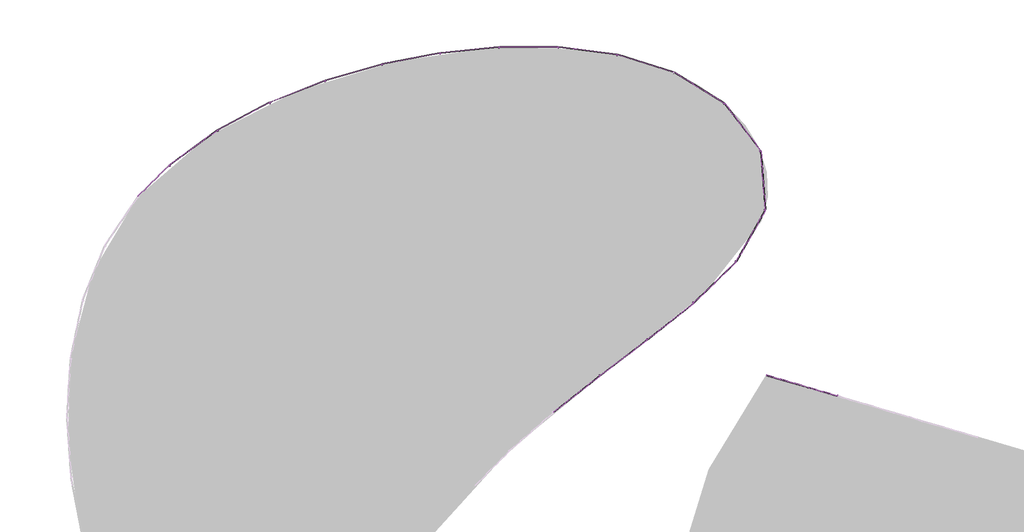
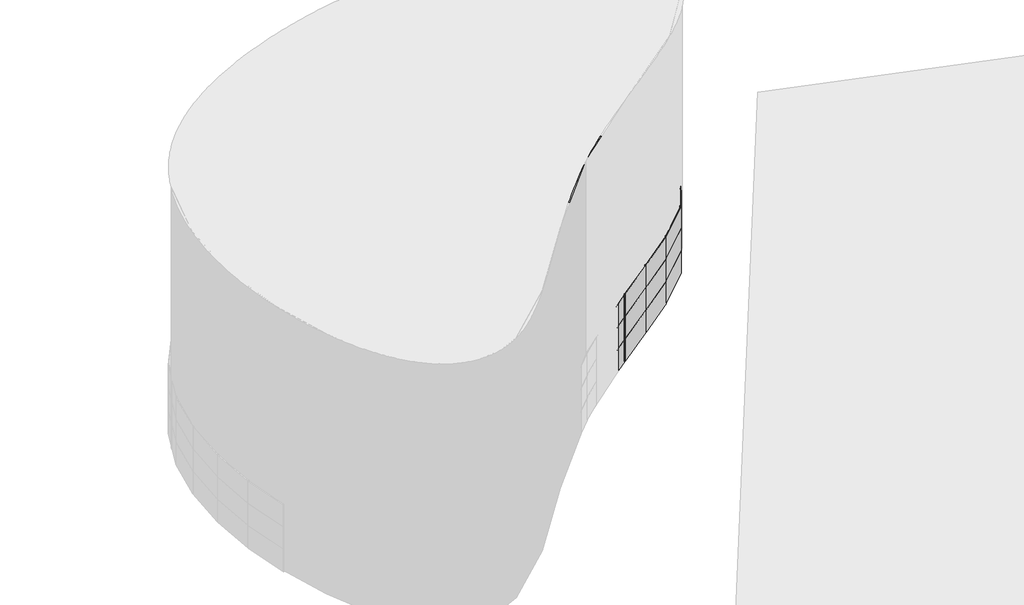
# One storey, part 4 of 5: 59 plates, 53 members.
"""IFC4 building model written with IfcOpenShell, lengths in millimetres."""

import ifcopenshell
import ifcopenshell.guid

model = None  # the IFC model being written
_history = None  # IfcOwnerHistory: only IFC2X3 demands one
_inside = {}  # id of a spatial element -> (the spatial element, [elements in it])
_under = {}  # id of a project, library or spatial element -> (it, [spatial elements below it])
_declared = {}  # id of a project -> (the project, [libraries it declares])
_typed = {}  # id of a type object -> (the type object, [elements of that type])
_made_of = {}  # id of a material, layer set ... -> (it, [elements and type objects made of it])


def new_model(schema):
    """Start an empty IFC model of exactly this schema.

    Asked for "IFC4X3", IfcOpenShell would pick the latest addendum, in which some entities
    have other attributes; the version numbers below select the first issue.
    IFC2X3 requires an IfcOwnerHistory on every rooted entity: one is made here for all.
    """
    global model, _history
    if schema == "IFC4X3":
        model = ifcopenshell.file(schema_version=(4, 3, 0, 0))
    else:
        model = ifcopenshell.file(schema=schema)
    _inside.clear()
    _under.clear()
    _declared.clear()
    _typed.clear()
    _made_of.clear()
    _history = None
    if model.schema == "IFC2X3":
        org = make("IfcOrganization", Name="unknown")
        user = make(
            "IfcPersonAndOrganization",
            ThePerson=make("IfcPerson", FamilyName="unknown"),
            TheOrganization=org,
        )
        app = make(
            "IfcApplication",
            ApplicationDeveloper=org,
            Version="unknown",
            ApplicationFullName="unknown",
            ApplicationIdentifier="unknown",
        )
        _history = make(
            "IfcOwnerHistory",
            OwningUser=user,
            OwningApplication=app,
            ChangeAction="ADDED",
            CreationDate=0,
        )
    return model


def make(cls, **values):
    """One entity of the class cls with the attributes given. An attribute that is None is left unset."""
    return model.create_entity(
        cls, **{name: value for name, value in values.items() if value is not None}
    )


def rooted(cls, **values):
    """An entity with a GlobalId (a new one), such as an element, a storey or a relation."""
    return make(cls, GlobalId=ifcopenshell.guid.new(), OwnerHistory=_history, **values)


def si_unit(unit_type, name, prefix=None):
    """IfcSIUnit, for example si_unit("LENGTHUNIT", "METRE", prefix="MILLI")."""
    return make("IfcSIUnit", UnitType=unit_type, Prefix=prefix, Name=name)


def assignment(units):
    """IfcUnitAssignment: the units of a project."""
    return None if units is None else make("IfcUnitAssignment", Units=units)


def point(xyz):
    """IfcCartesianPoint."""
    return None if xyz is None else make("IfcCartesianPoint", Coordinates=xyz)


def direction(xyz):
    """IfcDirection."""
    return None if xyz is None else make("IfcDirection", DirectionRatios=xyz)


def frame(location, z_axis=None, x_axis=None):
    """IfcAxis2Placement3D, a coordinate frame: its origin and axes. An axis left out is left unset."""
    return make(
        "IfcAxis2Placement3D",
        Location=point(location),
        Axis=direction(z_axis),
        RefDirection=direction(x_axis),
    )


def frame_2d(location, x_axis=None):
    """IfcAxis2Placement2D, a coordinate frame in the plane: its origin and x axis."""
    return make(
        "IfcAxis2Placement2D", Location=point(location), RefDirection=direction(x_axis)
    )


def origin():
    """The frame at (0, 0, 0) with its axes left unset."""
    return frame((0.0, 0.0, 0.0))


def origin_with_axes():
    """The frame at (0, 0, 0) with the z axis (0, 0, 1) and the x axis (1, 0, 0) written out."""
    return frame((0.0, 0.0, 0.0), z_axis=(0.0, 0.0, 1.0), x_axis=(1.0, 0.0, 0.0))


def origin_2d():
    """The frame at (0, 0) in the plane with its x axis left unset."""
    return frame_2d((0.0, 0.0))


def place(relative_to, where):
    """IfcLocalPlacement: puts the frame where relative to a parent placement (None: the world)."""
    return make(
        "IfcLocalPlacement", PlacementRelTo=relative_to, RelativePlacement=where
    )


def context(
    kind, dimensions, precision=None, world=None, true_north=None, identifier=None
):
    """IfcGeometricRepresentationContext, for example the 3D "Model" context."""
    return make(
        "IfcGeometricRepresentationContext",
        ContextIdentifier=identifier,
        ContextType=kind,
        CoordinateSpaceDimension=dimensions,
        Precision=precision,
        WorldCoordinateSystem=world,
        TrueNorth=true_north,
    )


def project(units=None, contexts=None):
    """IfcProject with its units and contexts."""
    return rooted(
        "IfcProject",
        Name="project",
        RepresentationContexts=contexts,
        UnitsInContext=assignment(units),
    )


def spatial(cls, under=None, at=None, **own):
    """A site, building, storey or space (cls), placed at a placement, below another one or the project."""
    s = rooted(cls, ObjectPlacement=at, **own)
    if under is not None:
        _under.setdefault(under.id(), (under, []))[1].append(s)
    return s


def polyline(points):
    """IfcPolyline through the points."""
    return make("IfcPolyline", Points=[point(p) for p in points])


def circle_curve(where, radius):
    """IfcCircle in the frame where."""
    return make("IfcCircle", Position=where, Radius=radius)


def trimmed(basis, trim1, trim2, sense, master):
    """IfcTrimmedCurve: the piece of a basis curve between two trims."""
    return make(
        "IfcTrimmedCurve",
        BasisCurve=basis,
        Trim1=trim1,
        Trim2=trim2,
        SenseAgreement=sense,
        MasterRepresentation=master,
    )


def segment(curve, same_sense, transition):
    """IfcCompositeCurveSegment."""
    return make(
        "IfcCompositeCurveSegment",
        Transition=transition,
        SameSense=same_sense,
        ParentCurve=curve,
    )


def composite_curve(segments, self_intersect=None):
    """IfcCompositeCurve: segments joined end to end."""
    return make("IfcCompositeCurve", Segments=segments, SelfIntersect=self_intersect)


def outline(outer, holes=None, kind="AREA"):
    """IfcArbitraryClosedProfileDef: a profile drawn as a closed curve; with holes, ...WithVoids."""
    if holes is None:
        return make("IfcArbitraryClosedProfileDef", ProfileType=kind, OuterCurve=outer)
    return make(
        "IfcArbitraryProfileDefWithVoids",
        ProfileType=kind,
        OuterCurve=outer,
        InnerCurves=holes,
    )


def extrude(swept, where, along, depth):
    """IfcExtrudedAreaSolid: the profile swept, set in the frame where, extruded along a direction by depth."""
    return make(
        "IfcExtrudedAreaSolid",
        SweptArea=swept,
        Position=where,
        ExtrudedDirection=direction(along),
        Depth=depth,
    )


def shape(context_of_items, identifier, shape_type, items):
    """IfcShapeRepresentation: the items that make up one representation, for example the "Body"."""
    return make(
        "IfcShapeRepresentation",
        ContextOfItems=context_of_items,
        RepresentationIdentifier=identifier,
        RepresentationType=shape_type,
        Items=items,
    )


def source(mapping_origin, context_of_items, identifier, shape_type, items):
    """IfcRepresentationMap: a shape defined once, which mapped items show again and again."""
    return make(
        "IfcRepresentationMap",
        MappingOrigin=mapping_origin,
        MappedRepresentation=shape(context_of_items, identifier, shape_type, items),
    )


def transform(
    local_origin,
    x_axis=None,
    y_axis=None,
    z_axis=None,
    scale=None,
    scale2=None,
    scale3=None,
    uniform=True,
):
    """IfcCartesianTransformationOperator3D, or its non-uniform kind. x_axis, y_axis, z_axis: its Axis1, 2, 3."""
    if uniform:
        return make(
            "IfcCartesianTransformationOperator3D",
            Axis1=direction(x_axis),
            Axis2=direction(y_axis),
            LocalOrigin=point(local_origin),
            Scale=scale,
            Axis3=direction(z_axis),
        )
    return make(
        "IfcCartesianTransformationOperator3DnonUniform",
        Axis1=direction(x_axis),
        Axis2=direction(y_axis),
        LocalOrigin=point(local_origin),
        Scale=scale,
        Axis3=direction(z_axis),
        Scale2=scale2,
        Scale3=scale3,
    )


def mapped(mapping_source, mapping_target):
    """IfcMappedItem: shows the shape of a source again, moved by a transform."""
    return make(
        "IfcMappedItem", MappingSource=mapping_source, MappingTarget=mapping_target
    )


def made_of(thing, what):
    """Note that an element or type object is made of a material, layer set ...; save() writes the relation."""
    if what is not None:
        _made_of.setdefault(what.id(), (what, []))[1].append(thing)
    return thing


def element(
    cls,
    number,
    at=None,
    inside=None,
    cuts=None,
    type_object=None,
    material=None,
    context=None,
    identifier="Body",
    shape_type=None,
    held_by="IfcProductDefinitionShape",
    body=None,
    shapes=None,
    **own,
):
    """One element of the class cls, such as IfcWall. Its Tag is "e" and its number.

    at: its placement. inside: the storey or other place that contains it. cuts: it is an
    opening in that element (IfcRelVoidsElement). A single representation is given by context,
    identifier, shape_type and body (its items); several are given by shapes. held_by: the class
    of the entity that holds the representations. save() writes the other relations.
    """
    e = rooted(cls, Tag="e%d" % number, ObjectPlacement=at, **own)
    if body is not None:
        shapes = [shape(context, identifier, shape_type, body)]
    if shapes is not None:
        e.Representation = make(held_by, Representations=shapes)
    if inside is not None:
        _inside.setdefault(inside.id(), (inside, []))[1].append(e)
    if cuts is not None:
        rooted(
            "IfcRelVoidsElement", RelatingBuildingElement=cuts, RelatedOpeningElement=e
        )
    if type_object is not None:
        _typed.setdefault(type_object.id(), (type_object, []))[1].append(e)
    return made_of(e, material)


def aggregate(whole, parts):
    """IfcRelAggregates: a whole, such as a stair, and the parts it consists of."""
    return rooted("IfcRelAggregates", RelatingObject=whole, RelatedObjects=parts)


def save(model, path):
    """Write the relations noted so far, then the file.

    IfcRelAggregates (storeys below a building ...), IfcRelContainedInSpatialStructure (elements
    in a storey), IfcRelDefinesByType, IfcRelAssociatesMaterial and IfcRelDeclares: one each for
    every whole, place, type object, material and project.
    """
    for whole, parts in _under.values():
        aggregate(whole, parts)
    for where, things in _inside.values():
        rooted(
            "IfcRelContainedInSpatialStructure",
            RelatedElements=things,
            RelatingStructure=where,
        )
    for kind, things in _typed.values():
        rooted("IfcRelDefinesByType", RelatedObjects=things, RelatingType=kind)
    for what, things in _made_of.values():
        rooted("IfcRelAssociatesMaterial", RelatedObjects=things, RelatingMaterial=what)
    for by, libraries in _declared.values():
        rooted("IfcRelDeclares", RelatingContext=by, RelatedDefinitions=libraries)
    model.write(path)


def montante_circular_25_mm_raio_36e581cf(model_context):
    return source(origin(), model_context, "Body", "SweptSolid", [
        extrude(outline(composite_curve([segment(trimmed(circle_curve(origin_2d(), 25.0), [point((25.0, 0.0))], [point((-25.0, 0.0))], False, "CARTESIAN"), True, "CONTINUOUS"), segment(trimmed(circle_curve(origin_2d(), 25.0), [point((-25.0, 0.0))], [point((25.0, 0.0))], False, "CARTESIAN"), True, "CONTINUOUS")], self_intersect=False)), frame((0.0, 0.0, -1500.0), z_axis=(0.0, 0.0, 1.0), x_axis=(1.0, 0.0, 0.0)), (0.0, 0.0, 1.0), 1500.0),
    ])


def montante_circular_25_mm_raio_a1f35a82(model_context):
    return source(origin(), model_context, "Body", "SweptSolid", [
        extrude(outline(composite_curve([segment(trimmed(circle_curve(origin_2d(), 25.0), [point((25.0, 0.0))], [point((-25.0, 0.0))], False, "CARTESIAN"), True, "CONTINUOUS"), segment(trimmed(circle_curve(origin_2d(), 25.0), [point((-25.0, 0.0))], [point((25.0, 0.0))], False, "CARTESIAN"), True, "CONTINUOUS")], self_intersect=False)), frame((0.0, 0.0, -727.4383788), z_axis=(0.0, 0.0, 1.0), x_axis=(1.0, 0.0, 0.0)), (0.0, 0.0, 1.0), 727.4383788),
    ])


def painel_do_sistema_ee4f1c4d(model_context):
    return source(origin(), model_context, "Body", "SweptSolid", [
        extrude(outline(polyline([(1487.5000075, 24.5), (-1487.5000075, 24.5), (-1487.5000075, 49.5), (1487.5000075, 49.5), (1487.5000075, 24.5)])), origin_with_axes(), (0.0, 0.0, 1.0), 1500.0),
    ])


def painel_do_sistema_5ef9eced(model_context):
    return source(origin(), model_context, "Body", "SweptSolid", [
        extrude(outline(polyline([(1475.0, 24.5), (-1475.0, 24.5), (-1475.0, 49.5), (1475.0, 49.5), (1475.0, 24.5)])), origin_with_axes(), (0.0, 0.0, 1.0), 1500.0),
    ])


def painel_do_sistema_cd1f443e(model_context):
    return source(origin(), model_context, "Body", "SweptSolid", [
        extrude(outline(polyline([(1487.5000075, 24.5), (-1487.5000075, 24.5), (-1487.5000075, 49.5), (1487.5000075, 49.5), (1487.5000075, 24.5)])), origin_with_axes(), (0.0, 0.0, 1.0), 727.4383788),
    ])


def painel_do_sistema_bf426e09(model_context):
    return source(origin(), model_context, "Body", "SweptSolid", [
        extrude(outline(polyline([(1475.0, 24.5), (-1475.0, 24.5), (-1475.0, 49.5), (1475.0, 49.5), (1475.0, 24.5)])), origin_with_axes(), (0.0, 0.0, 1.0), 727.4383788),
    ])


def painel_do_sistema_85ccde5d(model_context):
    return source(origin(), model_context, "Body", "SweptSolid", [
        extrude(outline(polyline([(1475.0, -49.5), (-1475.0, -49.5), (-1475.0, -24.5), (1475.0, -24.5), (1475.0, -49.5)])), origin_with_axes(), (0.0, 0.0, 1.0), 1500.0),
    ])


def painel_do_sistema_91df381f(model_context):
    return source(origin(), model_context, "Body", "SweptSolid", [
        extrude(outline(polyline([(1110.3819696, -49.5), (-1110.3819696, -49.5), (-1110.3819696, -24.5), (1110.3819696, -24.5), (1110.3819696, -49.5)])), origin_with_axes(), (0.0, 0.0, 1.0), 1500.0),
    ])


model = new_model("IFC4")

# Units and contexts
model_context = context("Model", 3, world=origin())
ifc_project = project(units=[si_unit("LENGTHUNIT", "METRE", prefix="MILLI")], contexts=[model_context])

# Site, building, storey
site = spatial("IfcSite", under=ifc_project)
building = spatial("IfcBuilding", under=site)
storey = spatial("IfcBuildingStorey", under=building, Name="Nível 1", Elevation=0.0)

# Members
placement = place(None, origin())
montante_circular_25_mm_raio_shape = montante_circular_25_mm_raio_36e581cf(model_context)
element("IfcMember", 1, ObjectType="Montante circular : 25 mm Raio", at=placement, inside=storey, context=model_context, shape_type="MappedRepresentation", body=[
    mapped(montante_circular_25_mm_raio_shape, transform((-4389.7681283, 32366.1480949, 3000.000015), x_axis=(0.0, 0.0, 1.0), y_axis=(0.28318378939534594, 0.95906566064253, 0.0), z_axis=(-0.95906566064253, 0.28318378939534594, 0.0))),
])
element("IfcMember", 2, ObjectType="Montante circular : 25 mm Raio", at=placement, inside=storey, context=model_context, shape_type="MappedRepresentation", body=[
    mapped(montante_circular_25_mm_raio_shape, transform((-5828.3666192, 32790.923779, 3000.000015), x_axis=(0.0, 0.0, 1.0), y_axis=(0.283183789395347, 0.9590656606425296, 0.0), z_axis=(-0.9590656606425296, 0.283183789395347, 0.0))),
])
element("IfcMember", 3, ObjectType="Montante circular : 25 mm Raio", at=placement, inside=storey, context=model_context, shape_type="MappedRepresentation", body=[
    mapped(montante_circular_25_mm_raio_shape, transform((-14996.1891623, 32974.6356945, 1500.0), x_axis=(0.7952150611070873, 0.6063274747102028, 0.0), y_axis=(0.6063274747102028, -0.7952150611070873, 0.0), z_axis=(0.0, 0.0, -1.0))),
])
element("IfcMember", 4, ObjectType="Montante circular : 25 mm Raio", at=placement, inside=storey, context=model_context, shape_type="MappedRepresentation", body=[
    mapped(montante_circular_25_mm_raio_shape, transform((-12604.1298635, 34785.1749266, 1500.0), x_axis=(0.7953870623365296, 0.6061018240095187, 0.0), y_axis=(0.6061018240095187, -0.7953870623365296, 0.0), z_axis=(0.0, 0.0, -1.0))),
])
element("IfcMember", 5, ObjectType="Montante circular : 25 mm Raio", at=placement, inside=storey, context=model_context, shape_type="MappedRepresentation", body=[
    mapped(montante_circular_25_mm_raio_shape, transform((-10255.474771, 36651.6741247, 1500.0), x_axis=(0.7627263023971693, 0.6467214142361005, 0.0), y_axis=(0.6467214142361005, -0.7627263023971693, 0.0), z_axis=(0.0, 0.0, -1.0))),
])
element("IfcMember", 6, ObjectType="Montante circular : 25 mm Raio", at=placement, inside=storey, context=model_context, shape_type="MappedRepresentation", body=[
    mapped(montante_circular_25_mm_raio_shape, transform((-8101.871437, 38740.2125323, 1500.0), x_axis=(0.6490334571140041, 0.7607598645739958, 0.0), y_axis=(0.7607598645739958, -0.6490334571140041, 0.0), z_axis=(0.0, 0.0, -1.0))),
])
element("IfcMember", 7, ObjectType="Montante circular : 25 mm Raio", at=placement, inside=storey, context=model_context, shape_type="MappedRepresentation", body=[
    mapped(montante_circular_25_mm_raio_shape, transform((-6627.5874319, 41352.9671461, 1500.0), x_axis=(0.24827563424230142, 0.9686894287859155, 0.0), y_axis=(0.9686894287859155, -0.24827563424230142, 0.0), z_axis=(0.0, 0.0, -1.0))),
])
element("IfcMember", 8, ObjectType="Montante circular : 25 mm Raio", at=placement, inside=storey, context=model_context, shape_type="MappedRepresentation", body=[
    mapped(montante_circular_25_mm_raio_shape, transform((-6868.5829053, 44343.271676, 1500.0), x_axis=(-0.3894872634933398, 0.9210318515537178, 0.0), y_axis=(0.9210318515537178, 0.3894872634933398, 0.0), z_axis=(0.0, 0.0, -1.0))),
])
element("IfcMember", 9, ObjectType="Montante circular : 25 mm Raio", at=placement, inside=storey, context=model_context, shape_type="MappedRepresentation", body=[
    mapped(montante_circular_25_mm_raio_shape, transform((-8685.5307871, 46730.4667655, 1500.0), x_axis=(-0.7608105002607383, 0.6489741001711895, 0.0), y_axis=(0.6489741001711895, 0.7608105002607383, 0.0), z_axis=(0.0, 0.0, -1.0))),
])
element("IfcMember", 10, ObjectType="Montante circular : 25 mm Raio", at=placement, inside=storey, context=model_context, shape_type="MappedRepresentation", body=[
    mapped(montante_circular_25_mm_raio_shape, transform((-11244.034472, 48297.0103794, 1500.0), x_axis=(-0.9160451113541028, 0.40107524725947563, 0.0), y_axis=(0.40107524725947563, 0.9160451113541028, 0.0), z_axis=(0.0, 0.0, -1.0))),
])
element("IfcMember", 11, ObjectType="Montante circular : 25 mm Raio", at=placement, inside=storey, context=model_context, shape_type="MappedRepresentation", body=[
    mapped(montante_circular_25_mm_raio_shape, transform((-14105.1754803, 49199.1589981, 1500.0), x_axis=(-0.9782677823869713, 0.20734547485700602, 0.0), y_axis=(0.20734547485700602, 0.9782677823869713, 0.0), z_axis=(0.0, 0.0, -1.0))),
])
element("IfcMember", 12, ObjectType="Montante circular : 25 mm Raio", at=placement, inside=storey, context=model_context, shape_type="MappedRepresentation", body=[
    mapped(montante_circular_25_mm_raio_shape, transform((-17080.2416106, 49585.140242, 1500.0), x_axis=(-0.998380379517221, 0.05689128048347721, 0.0), y_axis=(0.05689128048347721, 0.998380379517221, 0.0), z_axis=(0.0, 0.0, -1.0))),
])
element("IfcMember", 13, ObjectType="Montante circular : 25 mm Raio", at=placement, inside=storey, context=model_context, shape_type="MappedRepresentation", body=[
    mapped(montante_circular_25_mm_raio_shape, transform((-20080.239517, 49581.5960042, 1500.0), x_axis=(-0.9985092878419478, -0.054582067507252724, 0.0), y_axis=(-0.054582067507252724, 0.9985092878419478, 0.0), z_axis=(0.0, 0.0, -1.0))),
])
element("IfcMember", 14, ObjectType="Montante circular : 25 mm Raio", at=placement, inside=storey, context=model_context, shape_type="MappedRepresentation", body=[
    mapped(montante_circular_25_mm_raio_shape, transform((-23064.637889, 49276.0369149, 1500.0), x_axis=(-0.989112077587023, -0.14716418712269305, 0.0), y_axis=(-0.14716418712269305, 0.989112077587023, 0.0), z_axis=(0.0, 0.0, -1.0))),
])
element("IfcMember", 15, ObjectType="Montante circular : 25 mm Raio", at=placement, inside=storey, context=model_context, shape_type="MappedRepresentation", body=[
    mapped(montante_circular_25_mm_raio_shape, transform((-26009.7169515, 48704.6269783, 1500.0), x_axis=(-0.9724041864044524, -0.23330258949076227, 0.0), y_axis=(-0.23330258949076227, 0.9724041864044524, 0.0), z_axis=(0.0, 0.0, -1.0))),
])
element("IfcMember", 16, ObjectType="Montante circular : 25 mm Raio", at=placement, inside=storey, context=model_context, shape_type="MappedRepresentation", body=[
    mapped(montante_circular_25_mm_raio_shape, transform((-28892.5410808, 47874.3709699, 1500.0), x_axis=(-0.947152921337535, -0.3207823929111028, 0.0), y_axis=(-0.3207823929111028, 0.947152921337535, 0.0), z_axis=(0.0, 0.0, -1.0))),
])
element("IfcMember", 17, ObjectType="Montante circular : 25 mm Raio", at=placement, inside=storey, context=model_context, shape_type="MappedRepresentation", body=[
    mapped(montante_circular_25_mm_raio_shape, transform((-31682.4252949, 46771.3994961, 1500.0), x_axis=(-0.9093535544571357, -0.4160241735718888, 0.0), y_axis=(-0.4160241735718888, 0.9093535544571357, 0.0), z_axis=(0.0, 0.0, -1.0))),
])
element("IfcMember", 18, ObjectType="Montante circular : 25 mm Raio", at=placement, inside=storey, context=model_context, shape_type="MappedRepresentation", body=[
    mapped(montante_circular_25_mm_raio_shape, transform((-34331.1697585, 45362.7999198, 1500.0), x_axis=(-0.8509275894835548, -0.5252830070121313, 0.0), y_axis=(-0.5252830070121313, 0.8509275894835548, 0.0), z_axis=(0.0, 0.0, -1.0))),
])
element("IfcMember", 19, ObjectType="Montante circular : 25 mm Raio", at=placement, inside=storey, context=model_context, shape_type="MappedRepresentation", body=[
    mapped(montante_circular_25_mm_raio_shape, transform((-36756.8303499, 43597.5320378, 1500.0), x_axis=(-0.7567414762597636, -0.6537142633507346, 0.0), y_axis=(-0.6537142633507346, 0.7567414762597636, 0.0), z_axis=(0.0, 0.0, -1.0))),
])
element("IfcMember", 20, ObjectType="Montante circular : 25 mm Raio", at=placement, inside=storey, context=model_context, shape_type="MappedRepresentation", body=[
    mapped(montante_circular_25_mm_raio_shape, transform((-14996.1891623, 32974.6356945, 3000.0), x_axis=(0.7952150611070874, 0.6063274747102025, 0.0), y_axis=(0.6063274747102025, -0.7952150611070874, 0.0), z_axis=(0.0, 0.0, -1.0))),
])
element("IfcMember", 21, ObjectType="Montante circular : 25 mm Raio", at=placement, inside=storey, context=model_context, shape_type="MappedRepresentation", body=[
    mapped(montante_circular_25_mm_raio_shape, transform((-12604.1298635, 34785.1749266, 3000.0), x_axis=(0.7953870623365296, 0.6061018240095187, 0.0), y_axis=(0.6061018240095187, -0.7953870623365296, 0.0), z_axis=(0.0, 0.0, -1.0))),
])
element("IfcMember", 22, ObjectType="Montante circular : 25 mm Raio", at=placement, inside=storey, context=model_context, shape_type="MappedRepresentation", body=[
    mapped(montante_circular_25_mm_raio_shape, transform((-10255.474771, 36651.6741247, 3000.0), x_axis=(0.7627263023971692, 0.6467214142361006, 0.0), y_axis=(0.6467214142361006, -0.7627263023971692, 0.0), z_axis=(0.0, 0.0, -1.0))),
])
element("IfcMember", 23, ObjectType="Montante circular : 25 mm Raio", at=placement, inside=storey, context=model_context, shape_type="MappedRepresentation", body=[
    mapped(montante_circular_25_mm_raio_shape, transform((-8101.871437, 38740.2125323, 3000.0), x_axis=(0.6490334571140043, 0.7607598645739955, 0.0), y_axis=(0.7607598645739955, -0.6490334571140043, 0.0), z_axis=(0.0, 0.0, -1.0))),
])
element("IfcMember", 24, ObjectType="Montante circular : 25 mm Raio", at=placement, inside=storey, context=model_context, shape_type="MappedRepresentation", body=[
    mapped(montante_circular_25_mm_raio_shape, transform((-6627.5874319, 41352.9671461, 3000.0), x_axis=(0.24827563424230142, 0.9686894287859154, 0.0), y_axis=(0.9686894287859154, -0.24827563424230142, 0.0), z_axis=(0.0, 0.0, -1.0))),
])
element("IfcMember", 25, ObjectType="Montante circular : 25 mm Raio", at=placement, inside=storey, context=model_context, shape_type="MappedRepresentation", body=[
    mapped(montante_circular_25_mm_raio_shape, transform((-6868.5829053, 44343.271676, 3000.0), x_axis=(-0.3894872634933398, 0.9210318515537178, 0.0), y_axis=(0.9210318515537178, 0.3894872634933398, 0.0), z_axis=(0.0, 0.0, -1.0))),
])
element("IfcMember", 26, ObjectType="Montante circular : 25 mm Raio", at=placement, inside=storey, context=model_context, shape_type="MappedRepresentation", body=[
    mapped(montante_circular_25_mm_raio_shape, transform((-8685.5307871, 46730.4667655, 3000.0), x_axis=(-0.7608105002607387, 0.6489741001711892, 0.0), y_axis=(0.6489741001711892, 0.7608105002607387, 0.0), z_axis=(0.0, 0.0, -1.0))),
])
element("IfcMember", 27, ObjectType="Montante circular : 25 mm Raio", at=placement, inside=storey, context=model_context, shape_type="MappedRepresentation", body=[
    mapped(montante_circular_25_mm_raio_shape, transform((-14105.1754803, 49199.1589981, 3000.0), x_axis=(-0.9782677823869713, 0.20734547485700608, 0.0), y_axis=(0.20734547485700608, 0.9782677823869713, 0.0), z_axis=(0.0, 0.0, -1.0))),
])
element("IfcMember", 28, ObjectType="Montante circular : 25 mm Raio", at=placement, inside=storey, context=model_context, shape_type="MappedRepresentation", body=[
    mapped(montante_circular_25_mm_raio_shape, transform((-17080.2416106, 49585.140242, 3000.0), x_axis=(-0.998380379517221, 0.0568912804834772, 0.0), y_axis=(0.0568912804834772, 0.998380379517221, 0.0), z_axis=(0.0, 0.0, -1.0))),
])
element("IfcMember", 29, ObjectType="Montante circular : 25 mm Raio", at=placement, inside=storey, context=model_context, shape_type="MappedRepresentation", body=[
    mapped(montante_circular_25_mm_raio_shape, transform((-20080.239517, 49581.5960042, 3000.0), x_axis=(-0.9985092878419478, -0.05458206750725284, 0.0), y_axis=(-0.05458206750725284, 0.9985092878419478, 0.0), z_axis=(0.0, 0.0, -1.0))),
])
element("IfcMember", 30, ObjectType="Montante circular : 25 mm Raio", at=placement, inside=storey, context=model_context, shape_type="MappedRepresentation", body=[
    mapped(montante_circular_25_mm_raio_shape, transform((-23064.637889, 49276.0369149, 3000.0), x_axis=(-0.9891120775870231, -0.1471641871226927, 0.0), y_axis=(-0.1471641871226927, 0.9891120775870231, 0.0), z_axis=(0.0, 0.0, -1.0))),
])
element("IfcMember", 31, ObjectType="Montante circular : 25 mm Raio", at=placement, inside=storey, context=model_context, shape_type="MappedRepresentation", body=[
    mapped(montante_circular_25_mm_raio_shape, transform((-26009.7169515, 48704.6269783, 3000.0), x_axis=(-0.9724041864044525, -0.23330258949076174, 0.0), y_axis=(-0.23330258949076174, 0.9724041864044525, 0.0), z_axis=(0.0, 0.0, -1.0))),
])
element("IfcMember", 32, ObjectType="Montante circular : 25 mm Raio", at=placement, inside=storey, context=model_context, shape_type="MappedRepresentation", body=[
    mapped(montante_circular_25_mm_raio_shape, transform((-28892.5410808, 47874.3709699, 3000.0), x_axis=(-0.9471529213375351, -0.3207823929111028, 0.0), y_axis=(-0.3207823929111028, 0.9471529213375351, 0.0), z_axis=(0.0, 0.0, -1.0))),
])
element("IfcMember", 33, ObjectType="Montante circular : 25 mm Raio", at=placement, inside=storey, context=model_context, shape_type="MappedRepresentation", body=[
    mapped(montante_circular_25_mm_raio_shape, transform((-31682.4252949, 46771.3994961, 3000.0), x_axis=(-0.9093535544571357, -0.41602417357188887, 0.0), y_axis=(-0.41602417357188887, 0.9093535544571357, 0.0), z_axis=(0.0, 0.0, -1.0))),
])
element("IfcMember", 34, ObjectType="Montante circular : 25 mm Raio", at=placement, inside=storey, context=model_context, shape_type="MappedRepresentation", body=[
    mapped(montante_circular_25_mm_raio_shape, transform((-34331.1697585, 45362.7999198, 3000.0), x_axis=(-0.850927589483555, -0.5252830070121313, 0.0), y_axis=(-0.5252830070121313, 0.850927589483555, 0.0), z_axis=(0.0, 0.0, -1.0))),
])
element("IfcMember", 35, ObjectType="Montante circular : 25 mm Raio", at=placement, inside=storey, context=model_context, shape_type="MappedRepresentation", body=[
    mapped(montante_circular_25_mm_raio_shape, transform((-36756.8303499, 43597.5320378, 3000.0), x_axis=(-0.7567414762597636, -0.6537142633507346, 0.0), y_axis=(-0.6537142633507346, 0.7567414762597636, 0.0), z_axis=(0.0, 0.0, -1.0))),
])
montante_circular_25_mm_raio_2_shape = montante_circular_25_mm_raio_a1f35a82(model_context)
element("IfcMember", 36, ObjectType="Montante circular : 25 mm Raio", at=placement, inside=storey, context=model_context, shape_type="MappedRepresentation", body=[
    mapped(montante_circular_25_mm_raio_2_shape, transform((-6526.0277886, 32996.9225357, 3000.000015), x_axis=(0.0, 0.0, 1.0), y_axis=(0.28318378939534294, 0.9590656606425308, 0.0), z_axis=(-0.9590656606425308, 0.28318378939534294, 0.0))),
])
element("IfcMember", 37, ObjectType="Montante circular : 25 mm Raio", at=placement, inside=storey, context=model_context, shape_type="MappedRepresentation", body=[
    mapped(montante_circular_25_mm_raio_shape, transform((-14996.1891623, 32974.6356945, 0.0), x_axis=(0.7952150611070873, 0.6063274747102028, 0.0), y_axis=(0.6063274747102028, -0.7952150611070873, 0.0), z_axis=(0.0, 0.0, -1.0))),
])
element("IfcMember", 38, ObjectType="Montante circular : 25 mm Raio", at=placement, inside=storey, context=model_context, shape_type="MappedRepresentation", body=[
    mapped(montante_circular_25_mm_raio_shape, transform((-12604.1298635, 34785.1749266, 0.0), x_axis=(0.7953870623365296, 0.6061018240095187, 0.0), y_axis=(0.6061018240095187, -0.7953870623365296, 0.0), z_axis=(0.0, 0.0, -1.0))),
])
element("IfcMember", 39, ObjectType="Montante circular : 25 mm Raio", at=placement, inside=storey, context=model_context, shape_type="MappedRepresentation", body=[
    mapped(montante_circular_25_mm_raio_shape, transform((-10255.474771, 36651.6741247, 0.0), x_axis=(0.7627263023971693, 0.6467214142361005, 0.0), y_axis=(0.6467214142361005, -0.7627263023971693, 0.0), z_axis=(0.0, 0.0, -1.0))),
])
element("IfcMember", 40, ObjectType="Montante circular : 25 mm Raio", at=placement, inside=storey, context=model_context, shape_type="MappedRepresentation", body=[
    mapped(montante_circular_25_mm_raio_shape, transform((-8101.871437, 38740.2125323, 0.0), x_axis=(0.6490334571140042, 0.7607598645739956, 0.0), y_axis=(0.7607598645739956, -0.6490334571140042, 0.0), z_axis=(0.0, 0.0, -1.0))),
])
element("IfcMember", 41, ObjectType="Montante circular : 25 mm Raio", at=placement, inside=storey, context=model_context, shape_type="MappedRepresentation", body=[
    mapped(montante_circular_25_mm_raio_shape, transform((-6627.5874319, 41352.9671461, 0.0), x_axis=(0.24827563424230142, 0.9686894287859154, 0.0), y_axis=(0.9686894287859154, -0.24827563424230142, 0.0), z_axis=(0.0, 0.0, -1.0))),
])
element("IfcMember", 42, ObjectType="Montante circular : 25 mm Raio", at=placement, inside=storey, context=model_context, shape_type="MappedRepresentation", body=[
    mapped(montante_circular_25_mm_raio_shape, transform((-6868.5829053, 44343.271676, 0.0), x_axis=(-0.3894872634933398, 0.9210318515537178, 0.0), y_axis=(0.9210318515537178, 0.3894872634933398, 0.0), z_axis=(0.0, 0.0, -1.0))),
])
element("IfcMember", 43, ObjectType="Montante circular : 25 mm Raio", at=placement, inside=storey, context=model_context, shape_type="MappedRepresentation", body=[
    mapped(montante_circular_25_mm_raio_shape, transform((-8685.5307871, 46730.4667655, 0.0), x_axis=(-0.7608105002607386, 0.6489741001711892, 0.0), y_axis=(0.6489741001711892, 0.7608105002607386, 0.0), z_axis=(0.0, 0.0, -1.0))),
])
element("IfcMember", 44, ObjectType="Montante circular : 25 mm Raio", at=placement, inside=storey, context=model_context, shape_type="MappedRepresentation", body=[
    mapped(montante_circular_25_mm_raio_shape, transform((-11244.034472, 48297.0103794, 0.0), x_axis=(-0.9160451113541028, 0.40107524725947563, 0.0), y_axis=(0.40107524725947563, 0.9160451113541028, 0.0), z_axis=(0.0, 0.0, -1.0))),
])
element("IfcMember", 45, ObjectType="Montante circular : 25 mm Raio", at=placement, inside=storey, context=model_context, shape_type="MappedRepresentation", body=[
    mapped(montante_circular_25_mm_raio_shape, transform((-14105.1754803, 49199.1589981, 0.0), x_axis=(-0.9782677823869713, 0.20734547485700608, 0.0), y_axis=(0.20734547485700608, 0.9782677823869713, 0.0), z_axis=(0.0, 0.0, -1.0))),
])
element("IfcMember", 46, ObjectType="Montante circular : 25 mm Raio", at=placement, inside=storey, context=model_context, shape_type="MappedRepresentation", body=[
    mapped(montante_circular_25_mm_raio_shape, transform((-17080.2416106, 49585.140242, 0.0), x_axis=(-0.998380379517221, 0.0568912804834772, 0.0), y_axis=(0.0568912804834772, 0.998380379517221, 0.0), z_axis=(0.0, 0.0, -1.0))),
])
element("IfcMember", 47, ObjectType="Montante circular : 25 mm Raio", at=placement, inside=storey, context=model_context, shape_type="MappedRepresentation", body=[
    mapped(montante_circular_25_mm_raio_shape, transform((-20080.239517, 49581.5960042, 0.0), x_axis=(-0.9985092878419478, -0.05458206750725284, 0.0), y_axis=(-0.05458206750725284, 0.9985092878419478, 0.0), z_axis=(0.0, 0.0, -1.0))),
])
element("IfcMember", 48, ObjectType="Montante circular : 25 mm Raio", at=placement, inside=storey, context=model_context, shape_type="MappedRepresentation", body=[
    mapped(montante_circular_25_mm_raio_shape, transform((-23064.637889, 49276.0369149, 0.0), x_axis=(-0.9891120775870231, -0.14716418712269272, 0.0), y_axis=(-0.14716418712269272, 0.9891120775870231, 0.0), z_axis=(0.0, 0.0, -1.0))),
])
element("IfcMember", 49, ObjectType="Montante circular : 25 mm Raio", at=placement, inside=storey, context=model_context, shape_type="MappedRepresentation", body=[
    mapped(montante_circular_25_mm_raio_shape, transform((-26009.7169515, 48704.6269783, 0.0), x_axis=(-0.9724041864044524, -0.23330258949076224, 0.0), y_axis=(-0.23330258949076224, 0.9724041864044524, 0.0), z_axis=(0.0, 0.0, -1.0))),
])
element("IfcMember", 50, ObjectType="Montante circular : 25 mm Raio", at=placement, inside=storey, context=model_context, shape_type="MappedRepresentation", body=[
    mapped(montante_circular_25_mm_raio_shape, transform((-28892.5410808, 47874.3709699, 0.0), x_axis=(-0.9471529213375351, -0.3207823929111028, 0.0), y_axis=(-0.3207823929111028, 0.9471529213375351, 0.0), z_axis=(0.0, 0.0, -1.0))),
])
element("IfcMember", 51, ObjectType="Montante circular : 25 mm Raio", at=placement, inside=storey, context=model_context, shape_type="MappedRepresentation", body=[
    mapped(montante_circular_25_mm_raio_shape, transform((-31682.4252949, 46771.3994961, 0.0), x_axis=(-0.9093535544571357, -0.4160241735718888, 0.0), y_axis=(-0.4160241735718888, 0.9093535544571357, 0.0), z_axis=(0.0, 0.0, -1.0))),
])
element("IfcMember", 52, ObjectType="Montante circular : 25 mm Raio", at=placement, inside=storey, context=model_context, shape_type="MappedRepresentation", body=[
    mapped(montante_circular_25_mm_raio_shape, transform((-34331.1697585, 45362.7999198, 0.0), x_axis=(-0.850927589483555, -0.5252830070121313, 0.0), y_axis=(-0.5252830070121313, 0.850927589483555, 0.0), z_axis=(0.0, 0.0, -1.0))),
])
element("IfcMember", 53, ObjectType="Montante circular : 25 mm Raio", at=placement, inside=storey, context=model_context, shape_type="MappedRepresentation", body=[
    mapped(montante_circular_25_mm_raio_shape, transform((-36756.8303499, 43597.5320378, 0.0), x_axis=(-0.7567414762597636, -0.6537142633507346, 0.0), y_axis=(-0.6537142633507346, 0.7567414762597636, 0.0), z_axis=(0.0, 0.0, -1.0))),
])

# Plates
painel_do_sistema_shape = painel_do_sistema_ee4f1c4d(model_context)
element("IfcPlate", 54, ObjectType="Painel do sistema : Envidraçado", at=placement, inside=storey, context=model_context, shape_type="MappedRepresentation", body=[
    mapped(painel_do_sistema_shape, transform((-4389.7681283, 32366.1480949, 1487.5000075), x_axis=(0.0, 0.0, 1.0), y_axis=(-0.283183789395346, -0.95906566064253, 0.0), z_axis=(0.95906566064253, -0.283183789395346, 0.0))),
])
element("IfcPlate", 55, ObjectType="Painel do sistema : Envidraçado", at=placement, inside=storey, context=model_context, shape_type="MappedRepresentation", body=[
    mapped(painel_do_sistema_shape, transform((-5828.3666192, 32790.923779, 1487.5000075), x_axis=(0.0, 0.0, 1.0), y_axis=(-0.28318378939534705, -0.9590656606425296, 0.0), z_axis=(0.9590656606425296, -0.28318378939534705, 0.0))),
])
painel_do_sistema_2_shape = painel_do_sistema_5ef9eced(model_context)
element("IfcPlate", 56, ObjectType="Painel do sistema : Envidraçado", at=placement, inside=storey, context=model_context, shape_type="MappedRepresentation", body=[
    mapped(painel_do_sistema_2_shape, transform((-4389.7681283, 32366.1480949, 4500.00001), x_axis=(0.0, 0.0, 1.0), y_axis=(-0.283183789395346, -0.95906566064253, 0.0), z_axis=(0.95906566064253, -0.283183789395346, 0.0))),
])
element("IfcPlate", 57, ObjectType="Painel do sistema : Envidraçado", at=placement, inside=storey, context=model_context, shape_type="MappedRepresentation", body=[
    mapped(painel_do_sistema_2_shape, transform((-5828.3666192, 32790.923779, 4500.00001), x_axis=(0.0, 0.0, 1.0), y_axis=(-0.28318378939534705, -0.9590656606425297, 0.0), z_axis=(0.9590656606425297, -0.28318378939534705, 0.0))),
])
painel_do_sistema_3_shape = painel_do_sistema_cd1f443e(model_context)
element("IfcPlate", 58, ObjectType="Painel do sistema : Envidraçado", at=placement, inside=storey, context=model_context, shape_type="MappedRepresentation", body=[
    mapped(painel_do_sistema_3_shape, transform((-6526.0277886, 32996.9225357, 1487.5000075), x_axis=(0.0, 0.0, 1.0), y_axis=(-0.2831837893953438, -0.9590656606425306, 0.0), z_axis=(0.9590656606425306, -0.2831837893953438, 0.0))),
])
painel_do_sistema_4_shape = painel_do_sistema_bf426e09(model_context)
element("IfcPlate", 59, ObjectType="Painel do sistema : Envidraçado", at=placement, inside=storey, context=model_context, shape_type="MappedRepresentation", body=[
    mapped(painel_do_sistema_4_shape, transform((-6526.0277886, 32996.9225357, 4500.00001), x_axis=(0.0, 0.0, 1.0), y_axis=(-0.28318378939534383, -0.9590656606425306, 0.0), z_axis=(0.9590656606425306, -0.28318378939534383, 0.0))),
])
painel_do_sistema_5_shape = painel_do_sistema_85ccde5d(model_context)
element("IfcPlate", 60, ObjectType="Painel do sistema : Envidraçado", at=placement, inside=storey, context=model_context, shape_type="MappedRepresentation", body=[
    mapped(painel_do_sistema_5_shape, transform((-16174.7562692, 32046.745844, 0.0), x_axis=(0.7857114046077298, 0.6185932336110285, 0.0), y_axis=(-0.6185932336110285, 0.7857114046077298, 0.0), z_axis=(0.0, 0.0, 1.0))),
])
element("IfcPlate", 61, ObjectType="Painel do sistema : Envidraçado", at=placement, inside=storey, context=model_context, shape_type="MappedRepresentation", body=[
    mapped(painel_do_sistema_5_shape, transform((-13800.1595129, 33879.9053105, 0.0), x_axis=(0.7973530996033725, 0.6035130773669236, 0.0), y_axis=(-0.6035130773669236, 0.7973530996033725, 0.0), z_axis=(0.0, 0.0, 1.0))),
])
element("IfcPlate", 62, ObjectType="Painel do sistema : Envidraçado", at=placement, inside=storey, context=model_context, shape_type="MappedRepresentation", body=[
    mapped(painel_do_sistema_5_shape, transform((-11429.8023172, 35718.4245256, 0.0), x_axis=(0.7828850308262365, 0.6221663993725496, 0.0), y_axis=(-0.6221663993725496, 0.7828850308262365, 0.0), z_axis=(0.0, 0.0, 1.0))),
])
element("IfcPlate", 63, ObjectType="Painel do sistema : Envidraçado", at=placement, inside=storey, context=model_context, shape_type="MappedRepresentation", body=[
    mapped(painel_do_sistema_5_shape, transform((-9178.673104, 37695.9433285, 0.0), x_axis=(0.7178677779900101, 0.6961794691914476, 0.0), y_axis=(-0.6961794691914476, 0.7178677779900101, 0.0), z_axis=(0.0, 0.0, 1.0))),
])
element("IfcPlate", 64, ObjectType="Painel do sistema : Envidraçado", at=placement, inside=storey, context=model_context, shape_type="MappedRepresentation", body=[
    mapped(painel_do_sistema_5_shape, transform((-7364.7294344, 40046.5898392, 0.0), x_axis=(0.4914280017169703, 0.8709182046142253, 0.0), y_axis=(-0.8709182046142253, 0.4914280017169703, 0.0), z_axis=(0.0, 0.0, 1.0))),
])
element("IfcPlate", 65, ObjectType="Painel do sistema : Envidraçado", at=placement, inside=storey, context=model_context, shape_type="MappedRepresentation", body=[
    mapped(painel_do_sistema_5_shape, transform((-6748.0851686, 42848.1194111, 0.0), x_axis=(-0.08033182448940979, 0.9967681766460056, 0.0), y_axis=(-0.9967681766460056, -0.08033182448940979, 0.0), z_axis=(0.0, 0.0, 1.0))),
])
element("IfcPlate", 66, ObjectType="Painel do sistema : Envidraçado", at=placement, inside=storey, context=model_context, shape_type="MappedRepresentation", body=[
    mapped(painel_do_sistema_5_shape, transform((-7777.0568462, 45536.8692208, 0.0), x_axis=(-0.605649293912105, 0.7957316964805214, 0.0), y_axis=(-0.7957316964805214, -0.605649293912105, 0.0), z_axis=(0.0, 0.0, 1.0))),
])
element("IfcPlate", 67, ObjectType="Painel do sistema : Envidraçado", at=placement, inside=storey, context=model_context, shape_type="MappedRepresentation", body=[
    mapped(painel_do_sistema_5_shape, transform((-9964.7826295, 47513.7385724, 0.0), x_axis=(-0.8528345616365334, 0.5221812046389853, 0.0), y_axis=(-0.5221812046389853, -0.8528345616365334, 0.0), z_axis=(0.0, 0.0, 1.0))),
])
element("IfcPlate", 68, ObjectType="Painel do sistema : Envidraçado", at=placement, inside=storey, context=model_context, shape_type="MappedRepresentation", body=[
    mapped(painel_do_sistema_5_shape, transform((-12674.6049762, 48748.0846888, 0.0), x_axis=(-0.9537136694548438, 0.3007162062393329, 0.0), y_axis=(-0.3007162062393329, -0.9537136694548438, 0.0), z_axis=(0.0, 0.0, 1.0))),
])
element("IfcPlate", 69, ObjectType="Painel do sistema : Envidraçado", at=placement, inside=storey, context=model_context, shape_type="MappedRepresentation", body=[
    mapped(painel_do_sistema_5_shape, transform((-15592.7085455, 49392.1496201, 0.0), x_axis=(-0.9916887100842772, 0.12866041462463348, 0.0), y_axis=(-0.12866041462463348, -0.9916887100842772, 0.0), z_axis=(0.0, 0.0, 1.0))),
])
element("IfcPlate", 70, ObjectType="Painel do sistema : Envidraçado", at=placement, inside=storey, context=model_context, shape_type="MappedRepresentation", body=[
    mapped(painel_do_sistema_5_shape, transform((-18580.2405638, 49583.3681231, 0.0), x_axis=(-0.9999993021318769, -0.0011814126118296353, 0.0), y_axis=(0.0011814126118296353, -0.9999993021318769, 0.0), z_axis=(0.0, 0.0, 1.0))),
])
element("IfcPlate", 71, ObjectType="Painel do sistema : Envidraçado", at=placement, inside=storey, context=model_context, shape_type="MappedRepresentation", body=[
    mapped(painel_do_sistema_5_shape, transform((-21572.438703, 49428.8164595, 0.0), x_axis=(-0.9947994573422398, -0.10185302976144207, 0.0), y_axis=(0.10185302976144207, -0.9947994573422398, 0.0), z_axis=(0.0, 0.0, 1.0))),
])
element("IfcPlate", 72, ObjectType="Painel do sistema : Envidraçado", at=placement, inside=storey, context=model_context, shape_type="MappedRepresentation", body=[
    mapped(painel_do_sistema_5_shape, transform((-24537.1774203, 48990.3319466, 0.0), x_axis=(-0.9816930208347299, -0.1904699788533159, 0.0), y_axis=(0.1904699788533159, -0.9816930208347299, 0.0), z_axis=(0.0, 0.0, 1.0))),
])
element("IfcPlate", 73, ObjectType="Painel do sistema : Envidraçado", at=placement, inside=storey, context=model_context, shape_type="MappedRepresentation", body=[
    mapped(painel_do_sistema_5_shape, transform((-27451.1290162, 48289.4989741, 0.0), x_axis=(-0.9609413764383952, -0.2767520027907341, 0.0), y_axis=(0.2767520027907341, -0.9609413764383952, 0.0), z_axis=(0.0, 0.0, 1.0))),
])
element("IfcPlate", 74, ObjectType="Painel do sistema : Envidraçado", at=placement, inside=storey, context=model_context, shape_type="MappedRepresentation", body=[
    mapped(painel_do_sistema_5_shape, transform((-30287.4831879, 47322.885233, 0.0), x_axis=(-0.9299614046943586, -0.3676571579323536, 0.0), y_axis=(0.3676571579323536, -0.9299614046943586, 0.0), z_axis=(0.0, 0.0, 1.0))),
])
element("IfcPlate", 75, ObjectType="Painel do sistema : Envidraçado", at=placement, inside=storey, context=model_context, shape_type="MappedRepresentation", body=[
    mapped(painel_do_sistema_5_shape, transform((-33006.7975267, 46067.099708, 0.0), x_axis=(-0.8829148212020058, -0.46953319211939665, 0.0), y_axis=(0.46953319211939665, -0.8829148212020058, 0.0), z_axis=(0.0, 0.0, 1.0))),
])
element("IfcPlate", 76, ObjectType="Painel do sistema : Envidraçado", at=placement, inside=storey, context=model_context, shape_type="MappedRepresentation", body=[
    mapped(painel_do_sistema_5_shape, transform((-35544.0000542, 44480.1659788, 0.0), x_axis=(-0.8085535304668939, -0.5884226273432402, 0.0), y_axis=(0.5884226273432402, -0.8085535304668939, 0.0), z_axis=(0.0, 0.0, 1.0))),
])
element("IfcPlate", 77, ObjectType="Painel do sistema : Envidraçado", at=placement, inside=storey, context=model_context, shape_type="MappedRepresentation", body=[
    mapped(painel_do_sistema_5_shape, transform((-16174.7562692, 32046.745844, 1500.0), x_axis=(0.78571140460773, 0.6185932336110281, 0.0), y_axis=(-0.6185932336110281, 0.78571140460773, 0.0), z_axis=(0.0, 0.0, 1.0))),
])
element("IfcPlate", 78, ObjectType="Painel do sistema : Envidraçado", at=placement, inside=storey, context=model_context, shape_type="MappedRepresentation", body=[
    mapped(painel_do_sistema_5_shape, transform((-13800.1595129, 33879.9053105, 1500.0), x_axis=(0.7973530996033728, 0.6035130773669233, 0.0), y_axis=(-0.6035130773669233, 0.7973530996033728, 0.0), z_axis=(0.0, 0.0, 1.0))),
])
element("IfcPlate", 79, ObjectType="Painel do sistema : Envidraçado", at=placement, inside=storey, context=model_context, shape_type="MappedRepresentation", body=[
    mapped(painel_do_sistema_5_shape, transform((-11429.8023172, 35718.4245256, 1500.0), x_axis=(0.782885030826236, 0.6221663993725502, 0.0), y_axis=(-0.6221663993725502, 0.782885030826236, 0.0), z_axis=(0.0, 0.0, 1.0))),
])
element("IfcPlate", 80, ObjectType="Painel do sistema : Envidraçado", at=placement, inside=storey, context=model_context, shape_type="MappedRepresentation", body=[
    mapped(painel_do_sistema_5_shape, transform((-9178.673104, 37695.9433285, 1500.0), x_axis=(0.7178677779900108, 0.6961794691914469, 0.0), y_axis=(-0.6961794691914469, 0.7178677779900108, 0.0), z_axis=(0.0, 0.0, 1.0))),
])
element("IfcPlate", 81, ObjectType="Painel do sistema : Envidraçado", at=placement, inside=storey, context=model_context, shape_type="MappedRepresentation", body=[
    mapped(painel_do_sistema_5_shape, transform((-7364.7294344, 40046.5898392, 1500.0), x_axis=(0.4914280017169697, 0.8709182046142256, 0.0), y_axis=(-0.8709182046142256, 0.4914280017169697, 0.0), z_axis=(0.0, 0.0, 1.0))),
])
element("IfcPlate", 82, ObjectType="Painel do sistema : Envidraçado", at=placement, inside=storey, context=model_context, shape_type="MappedRepresentation", body=[
    mapped(painel_do_sistema_5_shape, transform((-6748.0851686, 42848.1194111, 1500.0), x_axis=(-0.08033182448940979, 0.9967681766460056, 0.0), y_axis=(-0.9967681766460056, -0.08033182448940979, 0.0), z_axis=(0.0, 0.0, 1.0))),
])
element("IfcPlate", 83, ObjectType="Painel do sistema : Envidraçado", at=placement, inside=storey, context=model_context, shape_type="MappedRepresentation", body=[
    mapped(painel_do_sistema_5_shape, transform((-7777.0568462, 45536.8692208, 1500.0), x_axis=(-0.605649293912105, 0.7957316964805214, 0.0), y_axis=(-0.7957316964805214, -0.605649293912105, 0.0), z_axis=(0.0, 0.0, 1.0))),
])
element("IfcPlate", 84, ObjectType="Painel do sistema : Envidraçado", at=placement, inside=storey, context=model_context, shape_type="MappedRepresentation", body=[
    mapped(painel_do_sistema_5_shape, transform((-9964.7826295, 47513.7385724, 1500.0), x_axis=(-0.8528345616365334, 0.5221812046389853, 0.0), y_axis=(-0.5221812046389853, -0.8528345616365334, 0.0), z_axis=(0.0, 0.0, 1.0))),
])
element("IfcPlate", 85, ObjectType="Painel do sistema : Envidraçado", at=placement, inside=storey, context=model_context, shape_type="MappedRepresentation", body=[
    mapped(painel_do_sistema_5_shape, transform((-12674.6049762, 48748.0846888, 1500.0), x_axis=(-0.9537136694548437, 0.30071620623933315, 0.0), y_axis=(-0.30071620623933315, -0.9537136694548437, 0.0), z_axis=(0.0, 0.0, 1.0))),
])
element("IfcPlate", 86, ObjectType="Painel do sistema : Envidraçado", at=placement, inside=storey, context=model_context, shape_type="MappedRepresentation", body=[
    mapped(painel_do_sistema_5_shape, transform((-15592.7085455, 49392.1496201, 1500.0), x_axis=(-0.9916887100842772, 0.12866041462463337, 0.0), y_axis=(-0.12866041462463337, -0.9916887100842772, 0.0), z_axis=(0.0, 0.0, 1.0))),
])
element("IfcPlate", 87, ObjectType="Painel do sistema : Envidraçado", at=placement, inside=storey, context=model_context, shape_type="MappedRepresentation", body=[
    mapped(painel_do_sistema_5_shape, transform((-18580.2405638, 49583.3681231, 1500.0), x_axis=(-0.9999993021318769, -0.0011814126118296353, 0.0), y_axis=(0.0011814126118296353, -0.9999993021318769, 0.0), z_axis=(0.0, 0.0, 1.0))),
])
element("IfcPlate", 88, ObjectType="Painel do sistema : Envidraçado", at=placement, inside=storey, context=model_context, shape_type="MappedRepresentation", body=[
    mapped(painel_do_sistema_5_shape, transform((-21572.438703, 49428.8164595, 1500.0), x_axis=(-0.9947994573422398, -0.10185302976144207, 0.0), y_axis=(0.10185302976144207, -0.9947994573422398, 0.0), z_axis=(0.0, 0.0, 1.0))),
])
element("IfcPlate", 89, ObjectType="Painel do sistema : Envidraçado", at=placement, inside=storey, context=model_context, shape_type="MappedRepresentation", body=[
    mapped(painel_do_sistema_5_shape, transform((-24537.1774203, 48990.3319466, 1500.0), x_axis=(-0.9816930208347299, -0.19046997885331615, 0.0), y_axis=(0.19046997885331615, -0.9816930208347299, 0.0), z_axis=(0.0, 0.0, 1.0))),
])
element("IfcPlate", 90, ObjectType="Painel do sistema : Envidraçado", at=placement, inside=storey, context=model_context, shape_type="MappedRepresentation", body=[
    mapped(painel_do_sistema_5_shape, transform((-27451.1290162, 48289.4989741, 1500.0), x_axis=(-0.9609413764383953, -0.2767520027907337, 0.0), y_axis=(0.2767520027907337, -0.9609413764383953, 0.0), z_axis=(0.0, 0.0, 1.0))),
])
element("IfcPlate", 91, ObjectType="Painel do sistema : Envidraçado", at=placement, inside=storey, context=model_context, shape_type="MappedRepresentation", body=[
    mapped(painel_do_sistema_5_shape, transform((-30287.4831879, 47322.885233, 1500.0), x_axis=(-0.9299614046943586, -0.3676571579323536, 0.0), y_axis=(0.3676571579323536, -0.9299614046943586, 0.0), z_axis=(0.0, 0.0, 1.0))),
])
element("IfcPlate", 92, ObjectType="Painel do sistema : Envidraçado", at=placement, inside=storey, context=model_context, shape_type="MappedRepresentation", body=[
    mapped(painel_do_sistema_5_shape, transform((-33006.7975267, 46067.099708, 1500.0), x_axis=(-0.8829148212020052, -0.46953319211939787, 0.0), y_axis=(0.46953319211939787, -0.8829148212020052, 0.0), z_axis=(0.0, 0.0, 1.0))),
])
element("IfcPlate", 93, ObjectType="Painel do sistema : Envidraçado", at=placement, inside=storey, context=model_context, shape_type="MappedRepresentation", body=[
    mapped(painel_do_sistema_5_shape, transform((-35544.0000542, 44480.1659788, 1500.0), x_axis=(-0.8085535304668945, -0.5884226273432396, 0.0), y_axis=(0.5884226273432396, -0.8085535304668945, 0.0), z_axis=(0.0, 0.0, 1.0))),
])
element("IfcPlate", 94, ObjectType="Painel do sistema : Envidraçado", at=placement, inside=storey, context=model_context, shape_type="MappedRepresentation", body=[
    mapped(painel_do_sistema_5_shape, transform((-16174.7562692, 32046.745844, 3000.0), x_axis=(0.7857114046077301, 0.6185932336110281, 0.0), y_axis=(-0.6185932336110281, 0.7857114046077301, 0.0), z_axis=(0.0, 0.0, 1.0))),
])
element("IfcPlate", 95, ObjectType="Painel do sistema : Envidraçado", at=placement, inside=storey, context=model_context, shape_type="MappedRepresentation", body=[
    mapped(painel_do_sistema_5_shape, transform((-13800.1595129, 33879.9053105, 3000.0), x_axis=(0.7973530996033725, 0.6035130773669236, 0.0), y_axis=(-0.6035130773669236, 0.7973530996033725, 0.0), z_axis=(0.0, 0.0, 1.0))),
])
element("IfcPlate", 96, ObjectType="Painel do sistema : Envidraçado", at=placement, inside=storey, context=model_context, shape_type="MappedRepresentation", body=[
    mapped(painel_do_sistema_5_shape, transform((-11429.8023172, 35718.4245256, 3000.0), x_axis=(0.7828850308262363, 0.6221663993725498, 0.0), y_axis=(-0.6221663993725498, 0.7828850308262363, 0.0), z_axis=(0.0, 0.0, 1.0))),
])
element("IfcPlate", 97, ObjectType="Painel do sistema : Envidraçado", at=placement, inside=storey, context=model_context, shape_type="MappedRepresentation", body=[
    mapped(painel_do_sistema_5_shape, transform((-9178.673104, 37695.9433285, 3000.0), x_axis=(0.7178677779900093, 0.6961794691914484, 0.0), y_axis=(-0.6961794691914484, 0.7178677779900093, 0.0), z_axis=(0.0, 0.0, 1.0))),
])
element("IfcPlate", 98, ObjectType="Painel do sistema : Envidraçado", at=placement, inside=storey, context=model_context, shape_type="MappedRepresentation", body=[
    mapped(painel_do_sistema_5_shape, transform((-7364.7294344, 40046.5898392, 3000.0), x_axis=(0.49142800171697093, 0.8709182046142249, 0.0), y_axis=(-0.8709182046142249, 0.49142800171697093, 0.0), z_axis=(0.0, 0.0, 1.0))),
])
element("IfcPlate", 99, ObjectType="Painel do sistema : Envidraçado", at=placement, inside=storey, context=model_context, shape_type="MappedRepresentation", body=[
    mapped(painel_do_sistema_5_shape, transform((-6748.0851686, 42848.1194111, 3000.0), x_axis=(-0.08033182448940979, 0.9967681766460056, 0.0), y_axis=(-0.9967681766460056, -0.08033182448940979, 0.0), z_axis=(0.0, 0.0, 1.0))),
])
element("IfcPlate", 100, ObjectType="Painel do sistema : Envidraçado", at=placement, inside=storey, context=model_context, shape_type="MappedRepresentation", body=[
    mapped(painel_do_sistema_5_shape, transform((-7777.0568462, 45536.8692208, 3000.0), x_axis=(-0.605649293912105, 0.7957316964805214, 0.0), y_axis=(-0.7957316964805214, -0.605649293912105, 0.0), z_axis=(0.0, 0.0, 1.0))),
])
element("IfcPlate", 101, ObjectType="Painel do sistema : Envidraçado", at=placement, inside=storey, context=model_context, shape_type="MappedRepresentation", body=[
    mapped(painel_do_sistema_5_shape, transform((-9964.7826295, 47513.7385724, 3000.0), x_axis=(-0.8528345616365334, 0.5221812046389853, 0.0), y_axis=(-0.5221812046389853, -0.8528345616365334, 0.0), z_axis=(0.0, 0.0, 1.0))),
])
element("IfcPlate", 102, ObjectType="Painel do sistema : Envidraçado", at=placement, inside=storey, context=model_context, shape_type="MappedRepresentation", body=[
    mapped(painel_do_sistema_5_shape, transform((-12674.6049762, 48748.0846888, 3000.0), x_axis=(-0.9537136694548437, 0.30071620623933315, 0.0), y_axis=(-0.30071620623933315, -0.9537136694548437, 0.0), z_axis=(0.0, 0.0, 1.0))),
])
element("IfcPlate", 103, ObjectType="Painel do sistema : Envidraçado", at=placement, inside=storey, context=model_context, shape_type="MappedRepresentation", body=[
    mapped(painel_do_sistema_5_shape, transform((-15592.7085455, 49392.1496201, 3000.0), x_axis=(-0.9916887100842772, 0.12866041462463337, 0.0), y_axis=(-0.12866041462463337, -0.9916887100842772, 0.0), z_axis=(0.0, 0.0, 1.0))),
])
element("IfcPlate", 104, ObjectType="Painel do sistema : Envidraçado", at=placement, inside=storey, context=model_context, shape_type="MappedRepresentation", body=[
    mapped(painel_do_sistema_5_shape, transform((-18580.2405638, 49583.3681231, 3000.0), x_axis=(-0.9999993021318769, -0.0011814126118296353, 0.0), y_axis=(0.0011814126118296353, -0.9999993021318769, 0.0), z_axis=(0.0, 0.0, 1.0))),
])
element("IfcPlate", 105, ObjectType="Painel do sistema : Envidraçado", at=placement, inside=storey, context=model_context, shape_type="MappedRepresentation", body=[
    mapped(painel_do_sistema_5_shape, transform((-21572.438703, 49428.8164595, 3000.0), x_axis=(-0.9947994573422398, -0.10185302976144207, 0.0), y_axis=(0.10185302976144207, -0.9947994573422398, 0.0), z_axis=(0.0, 0.0, 1.0))),
])
element("IfcPlate", 106, ObjectType="Painel do sistema : Envidraçado", at=placement, inside=storey, context=model_context, shape_type="MappedRepresentation", body=[
    mapped(painel_do_sistema_5_shape, transform((-24537.1774203, 48990.3319466, 3000.0), x_axis=(-0.9816930208347299, -0.1904699788533159, 0.0), y_axis=(0.1904699788533159, -0.9816930208347299, 0.0), z_axis=(0.0, 0.0, 1.0))),
])
element("IfcPlate", 107, ObjectType="Painel do sistema : Envidraçado", at=placement, inside=storey, context=model_context, shape_type="MappedRepresentation", body=[
    mapped(painel_do_sistema_5_shape, transform((-27451.1290162, 48289.4989741, 3000.0), x_axis=(-0.9609413764383952, -0.2767520027907341, 0.0), y_axis=(0.2767520027907341, -0.9609413764383952, 0.0), z_axis=(0.0, 0.0, 1.0))),
])
element("IfcPlate", 108, ObjectType="Painel do sistema : Envidraçado", at=placement, inside=storey, context=model_context, shape_type="MappedRepresentation", body=[
    mapped(painel_do_sistema_5_shape, transform((-30287.4831879, 47322.885233, 3000.0), x_axis=(-0.9299614046943586, -0.36765715793235343, 0.0), y_axis=(0.36765715793235343, -0.9299614046943586, 0.0), z_axis=(0.0, 0.0, 1.0))),
])
element("IfcPlate", 109, ObjectType="Painel do sistema : Envidraçado", at=placement, inside=storey, context=model_context, shape_type="MappedRepresentation", body=[
    mapped(painel_do_sistema_5_shape, transform((-33006.7975267, 46067.099708, 3000.0), x_axis=(-0.8829148212020055, -0.46953319211939715, 0.0), y_axis=(0.46953319211939715, -0.8829148212020055, 0.0), z_axis=(0.0, 0.0, 1.0))),
])
element("IfcPlate", 110, ObjectType="Painel do sistema : Envidraçado", at=placement, inside=storey, context=model_context, shape_type="MappedRepresentation", body=[
    mapped(painel_do_sistema_5_shape, transform((-35544.0000542, 44480.1659788, 3000.0), x_axis=(-0.8085535304668939, -0.5884226273432402, 0.0), y_axis=(0.5884226273432402, -0.8085535304668939, 0.0), z_axis=(0.0, 0.0, 1.0))),
])
painel_do_sistema_6_shape = painel_do_sistema_91df381f(model_context)
element("IfcPlate", 111, ObjectType="Painel do sistema : Envidraçado", at=placement, inside=storey, context=model_context, shape_type="MappedRepresentation", body=[
    mapped(painel_do_sistema_6_shape, transform((-37558.9942636, 42794.0239341, 1500.0), x_axis=(-0.7065145784499645, -0.7076984883675174, 0.0), y_axis=(0.7076984883675174, -0.7065145784499645, 0.0), z_axis=(0.0, 0.0, 1.0))),
])
element("IfcPlate", 112, ObjectType="Painel do sistema : Envidraçado", at=placement, inside=storey, context=model_context, shape_type="MappedRepresentation", body=[
    mapped(painel_do_sistema_6_shape, transform((-37558.9942636, 42794.0239341, 3000.0), x_axis=(-0.7065145784499645, -0.7076984883675173, 0.0), y_axis=(0.7076984883675173, -0.7065145784499645, 0.0), z_axis=(0.0, 0.0, 1.0))),
])

save(model, "model.ifc")

# Revit data of these elements
# Type "Montante circular : 25 mm Raio"
#   built-in parameter 1007350 = 0.082021 (stored number, unit not read)
# Type "Painel do sistema : Envidraçado"
#   Construction Type Id = "GSP4R"
#   Analytic Construction = "Vidraça única Pilkington 1/8 pol"
#   Visual Light Transmittance = 0.9
#   Solar Heat Gain Coefficient = 0.86
#   Heat Transfer Coefficient (U) = 6.7069 W/(m²·K)
# Elements 1, 2, 3, 4, 5, 6, 7, 8, 9, 10, 11, 12, 13, 14, 15, 16, 17, 18, 19, 20, 21, 22, 23, 24, 25, 26, 27, 28, 29, 30, 31, 32, 33, 34, 35, 36, 37, 38, 39, 40, 41, 42, 43, 44, 45, 46, 47, 48, 49, 50, 51, 52, 53 (IfcMember, "Montante circular : 25 mm Raio")
#   Phase Created = Construção nova
#   Materials on its faces: "Alumín."
# Elements 54, 55, 56, 57, 58, 59, 60, 61, 62, 63, 64, 65, 66, 67, 68, 69, 70, 71, 72, 73, 74, 75, 76, 77, 78, 79, 80, 81, 82, 83, 84, 85, 86, 87, 88, 89, 90, 91, 92, 93, 94, 95, 96, 97, 98, 99, 100, 101, 102, 103, 104, 105, 106, 107, 108, 109, 110, 111, 112 (IfcPlate, "Painel do sistema : Envidraçado")
#   Phase Created = Construção nova
#   Materials on its faces: "Vidro"
# Materials
#   "Alumín.": class "Metal", colour RGB 247 247 247, transparency 0, Description = "Alumín. 6061", Cost = 0
#   "Vidro": class "Vidro", colour RGB 0 128 192, transparency 0.9, Description = "Vidro de sílica", Cost = 0
